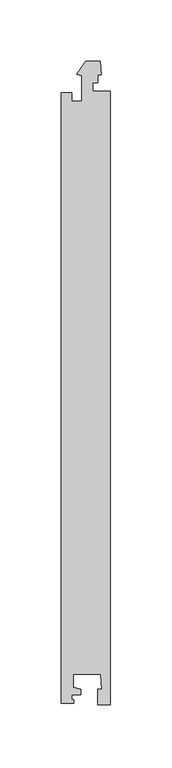
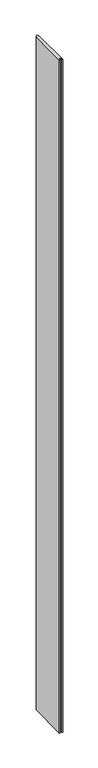
"""IFC4 building model written with IfcOpenShell, lengths in millimetres: proxy geometry, Generic Models 5:Generic Models 5:321804:Generic Models 5:321804 : Generic Models 5:Generic Models 5:321804:35 : Generic Models 5:Generic Models 5:321804:Generic Models 5:321804 : Generic Models 5:Generic Models 5:321804:300761."""

from ifc_helpers import new_model, si_unit, frame, origin, place, context, project, spatial, polyline, outline, extrude, source, transform, mapped, element, save


def generic_models_bd2a6c0a(model_context):
    return source(origin(), model_context, "Body", "SweptSolid", [
        extrude(outline(polyline([(667625.2338797, -491910.833465), (667631.7338797, -491912.5751348), (667631.7338797, -491917.0251348), (667624.2338797, -491917.0251348), (667624.2338797, -491920.9751348), (667625.7338797, -491920.9751348), (667625.7338797, -491923.9751348), (667615.7338797, -491923.9751348), (667615.7338797, -491426.4751348), (667624.2338797, -491426.4751348), (667624.2338797, -491433.4251348), (667632.2338797, -491433.4251348), (667632.2338797, -491412.7091094), (667628.3059983, -491411.6566367), (667635.4133634, -491400.9751348), (667647.2715044, -491400.9751348), (667648.2338797, -491411.9751348), (667645.5338797, -491411.9751348), (667645.5338797, -491418.6001348), (667641.2338797, -491418.6001348), (667641.2338797, -491425.2251348), (667655.7338797, -491425.2251348), (667655.7338797, -491925.2251348), (667645.5338797, -491925.2251348), (667645.5338797, -491912.4751348), (667648.779534, -491912.4751348), (667647.72967, -491900.4751348), (667625.2338797, -491900.4751348), (667625.2338797, -491910.833465)])), frame((0.0, 0.0, -5.8417589), z_axis=(0.0, 0.0, 1.0), x_axis=(1.0, 0.0, 0.0)), (0.0, 0.0, 1.0), 8779.7126309),
    ])


if __name__ == "__main__":
    model = new_model("IFC4")
    model_context = context("Model", 3, world=origin())
    ifc_project = project(units=[si_unit("LENGTHUNIT", "METRE", prefix="MILLI")], contexts=[model_context])
    site = spatial("IfcSite", under=ifc_project)
    building = spatial("IfcBuilding", under=site)
    placement = place(None, origin())
    generic_models_shape = generic_models_bd2a6c0a(model_context)
    element("IfcBuildingElementProxy", 1, Name="Generic Models 5:Generic Models 5:321804:Generic Models 5:321804 : Generic Models 5:Generic Models 5:321804:35 : Generic Models 5:Generic Models 5:321804:Generic Models 5:321804 : Generic Models 5:Generic Models 5:321804:300761", ObjectType="Generic Models 5:Generic Models 5:321804:Generic Models 5:321804 : Generic Models 5:Generic Models 5:321804:35 : Generic Models 5:Generic Models 5:321804:Generic Models 5:321804 : Generic Models 5:Generic Models 5:321804:300761", at=placement, inside=building, context=model_context, shape_type="MappedRepresentation", body=[
        mapped(generic_models_shape, transform((0.0, 0.0, 0.0), x_axis=(1.0, 0.0, 0.0), y_axis=(0.0, 1.0, 0.0), z_axis=(0.0, 0.0, 1.0))),
    ])
    save(model, "model.ifc")

# Revit data of these elements
# Type "Generic Models 5:Generic Models 5:321804:Generic Models 5:321804 : Generic Models 5:Generic Models 5:321804:35 : Generic Models 5:Generic Models 5:321804:Generic Models 5:321804 : Generic Models 5:Generic Models 5:321804:300761"
#   NameOverride = "Generic Models 5:Generic Models 5:321804:Generic Models 5:321804 : Generic Models 5:Generic Models 5:321804:300761"
#   ObjectTypeOverride = "Generic Models 5:321804 : Generic Models 5:Generic Models 5:321804"
#   Reference = "Generic Models 5"
#   Tag = "300761"
# Element 1 (IfcBuildingElementProxy, "Generic Models 5:Generic Models 5:321804:Generic Models 5:321804 : Generic Models 5:Generic Models 5:321804:35 : Generic Models 5:Generic Models 5:321804:Generic Models 5:321804 : Generic Models 5:Generic Models 5:321804:300761")
#   Materials on its faces: "POLYCARBONATE PANEL - ARCOPLUS 547"
# Materials
#   "POLYCARBONATE PANEL - ARCOPLUS 547": class "Unassigned", colour RGB 202 225 249, transparency 0.45, Cost = 0
